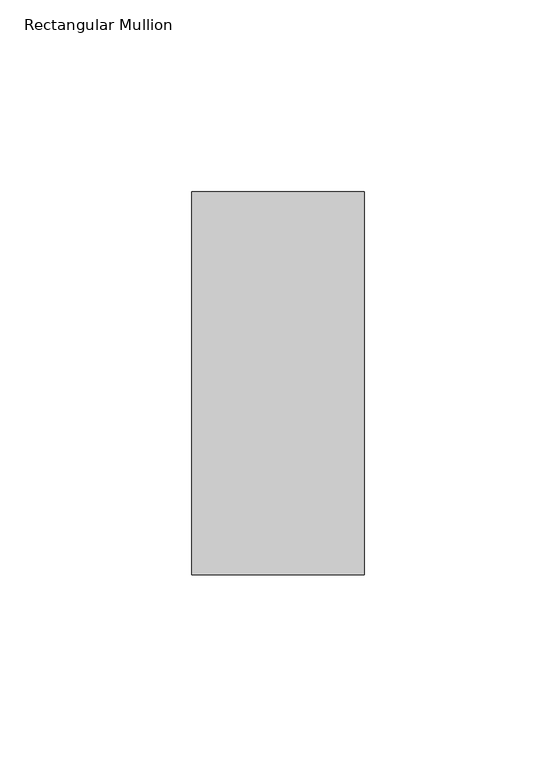
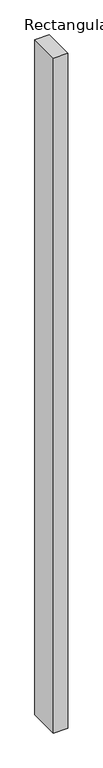
"""IFC4 building model written with IfcOpenShell, lengths in millimetres: member geometry, Rectangular Mullion : 알루미늄_Rectangular Cap_100 x 45."""

from ifc_helpers import new_model, si_unit, frame, origin, place, context, project, spatial, polyline, outline, extrude, source, transform, mapped, element, save


def rectangular_mullion_c5c797fa(model_context):
    return source(origin(), model_context, "Body", "SweptSolid", [
        extrude(outline(polyline([(0.0, 50.0), (0.0, -50.0), (-45.0, -50.0), (-45.0, 50.0), (0.0, 50.0)])), frame((0.0, 0.0, -2222.5), z_axis=(0.0, 0.0, 1.0), x_axis=(1.0, 0.0, 0.0)), (0.0, 0.0, 1.0), 2222.5),
    ])


if __name__ == "__main__":
    model = new_model("IFC4")
    model_context = context("Model", 3, world=origin())
    ifc_project = project(units=[si_unit("LENGTHUNIT", "METRE", prefix="MILLI")], contexts=[model_context])
    site = spatial("IfcSite", under=ifc_project)
    building = spatial("IfcBuilding", under=site)
    placement = place(None, origin())
    rectangular_mullion_shape = rectangular_mullion_c5c797fa(model_context)
    element("IfcMember", 1, ObjectType="Rectangular Mullion : 알루미늄_Rectangular Cap_100 x 45", at=placement, inside=building, context=model_context, shape_type="MappedRepresentation", body=[
        mapped(rectangular_mullion_shape, transform((0.0, 0.0, 0.0), x_axis=(1.0, 0.0, 0.0), y_axis=(0.0, 1.0, 0.0), z_axis=(0.0, 0.0, 1.0))),
    ])
    save(model, "model.ifc")

# Revit data of these elements
# Type "Rectangular Mullion : 알루미늄_Rectangular Cap_100 x 45"
#   built-in parameter 1007304 = 0.328084 (stored number, unit not read)
#   built-in parameter 1007301 = 0.0738189 (stored number, unit not read)
#   built-in parameter 1007300 = 0.0738189 (stored number, unit not read)
# Element 1 (IfcMember, "Rectangular Mullion : 알루미늄_Rectangular Cap_100 x 45")
#   Materials on its faces: "00_Metal_Stainless Steel"
# Materials
#   "00_Metal_Stainless Steel": class "Metal", colour RGB 148 148 148, transparency 0, Description = "Steel", Cost = 0
